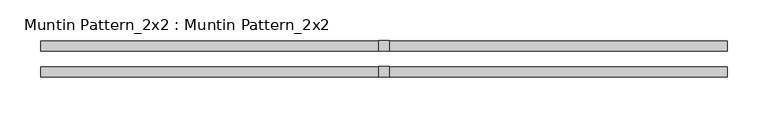
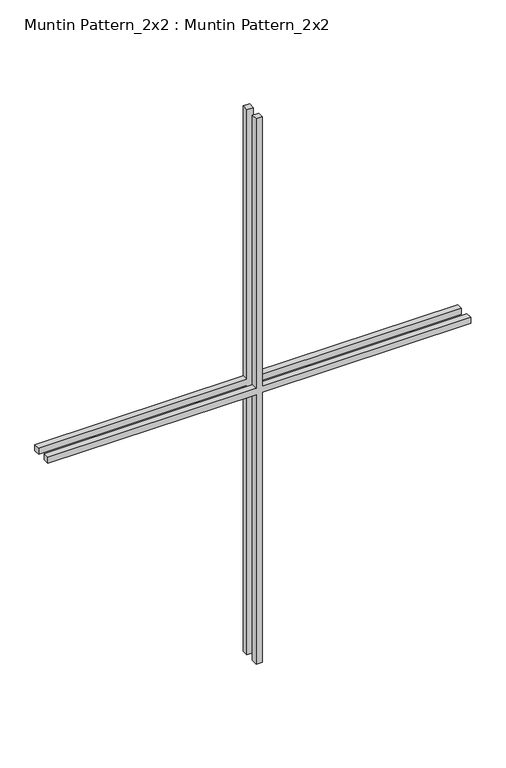
"""IFC4 building model written with IfcOpenShell, lengths in millimetres: proxy geometry, Muntin Pattern_2x2 : Muntin Pattern_2x2."""

import ifcopenshell
import ifcopenshell.guid

model = None  # the IFC model being written
_history = None  # IfcOwnerHistory: only IFC2X3 demands one
_inside = {}  # id of a spatial element -> (the spatial element, [elements in it])
_under = {}  # id of a project, library or spatial element -> (it, [spatial elements below it])
_declared = {}  # id of a project -> (the project, [libraries it declares])
_typed = {}  # id of a type object -> (the type object, [elements of that type])
_made_of = {}  # id of a material, layer set ... -> (it, [elements and type objects made of it])


def new_model(schema):
    """Start an empty IFC model of exactly this schema.

    Asked for "IFC4X3", IfcOpenShell would pick the latest addendum, in which some entities
    have other attributes; the version numbers below select the first issue.
    IFC2X3 requires an IfcOwnerHistory on every rooted entity: one is made here for all.
    """
    global model, _history
    if schema == "IFC4X3":
        model = ifcopenshell.file(schema_version=(4, 3, 0, 0))
    else:
        model = ifcopenshell.file(schema=schema)
    _inside.clear()
    _under.clear()
    _declared.clear()
    _typed.clear()
    _made_of.clear()
    _history = None
    if model.schema == "IFC2X3":
        org = make("IfcOrganization", Name="unknown")
        user = make(
            "IfcPersonAndOrganization",
            ThePerson=make("IfcPerson", FamilyName="unknown"),
            TheOrganization=org,
        )
        app = make(
            "IfcApplication",
            ApplicationDeveloper=org,
            Version="unknown",
            ApplicationFullName="unknown",
            ApplicationIdentifier="unknown",
        )
        _history = make(
            "IfcOwnerHistory",
            OwningUser=user,
            OwningApplication=app,
            ChangeAction="ADDED",
            CreationDate=0,
        )
    return model


def make(cls, **values):
    """One entity of the class cls with the attributes given. An attribute that is None is left unset."""
    return model.create_entity(
        cls, **{name: value for name, value in values.items() if value is not None}
    )


def rooted(cls, **values):
    """An entity with a GlobalId (a new one), such as an element, a storey or a relation."""
    return make(cls, GlobalId=ifcopenshell.guid.new(), OwnerHistory=_history, **values)


def si_unit(unit_type, name, prefix=None):
    """IfcSIUnit, for example si_unit("LENGTHUNIT", "METRE", prefix="MILLI")."""
    return make("IfcSIUnit", UnitType=unit_type, Prefix=prefix, Name=name)


def assignment(units):
    """IfcUnitAssignment: the units of a project."""
    return None if units is None else make("IfcUnitAssignment", Units=units)


def point(xyz):
    """IfcCartesianPoint."""
    return None if xyz is None else make("IfcCartesianPoint", Coordinates=xyz)


def direction(xyz):
    """IfcDirection."""
    return None if xyz is None else make("IfcDirection", DirectionRatios=xyz)


def frame(location, z_axis=None, x_axis=None):
    """IfcAxis2Placement3D, a coordinate frame: its origin and axes. An axis left out is left unset."""
    return make(
        "IfcAxis2Placement3D",
        Location=point(location),
        Axis=direction(z_axis),
        RefDirection=direction(x_axis),
    )


def origin():
    """The frame at (0, 0, 0) with its axes left unset."""
    return frame((0.0, 0.0, 0.0))


def place(relative_to, where):
    """IfcLocalPlacement: puts the frame where relative to a parent placement (None: the world)."""
    return make(
        "IfcLocalPlacement", PlacementRelTo=relative_to, RelativePlacement=where
    )


def context(
    kind, dimensions, precision=None, world=None, true_north=None, identifier=None
):
    """IfcGeometricRepresentationContext, for example the 3D "Model" context."""
    return make(
        "IfcGeometricRepresentationContext",
        ContextIdentifier=identifier,
        ContextType=kind,
        CoordinateSpaceDimension=dimensions,
        Precision=precision,
        WorldCoordinateSystem=world,
        TrueNorth=true_north,
    )


def project(units=None, contexts=None):
    """IfcProject with its units and contexts."""
    return rooted(
        "IfcProject",
        Name="project",
        RepresentationContexts=contexts,
        UnitsInContext=assignment(units),
    )


def spatial(cls, under=None, at=None, **own):
    """A site, building, storey or space (cls), placed at a placement, below another one or the project."""
    s = rooted(cls, ObjectPlacement=at, **own)
    if under is not None:
        _under.setdefault(under.id(), (under, []))[1].append(s)
    return s


def polyline(points):
    """IfcPolyline through the points."""
    return make("IfcPolyline", Points=[point(p) for p in points])


def outline(outer, holes=None, kind="AREA"):
    """IfcArbitraryClosedProfileDef: a profile drawn as a closed curve; with holes, ...WithVoids."""
    if holes is None:
        return make("IfcArbitraryClosedProfileDef", ProfileType=kind, OuterCurve=outer)
    return make(
        "IfcArbitraryProfileDefWithVoids",
        ProfileType=kind,
        OuterCurve=outer,
        InnerCurves=holes,
    )


def extrude(swept, where, along, depth):
    """IfcExtrudedAreaSolid: the profile swept, set in the frame where, extruded along a direction by depth."""
    return make(
        "IfcExtrudedAreaSolid",
        SweptArea=swept,
        Position=where,
        ExtrudedDirection=direction(along),
        Depth=depth,
    )


def shape(context_of_items, identifier, shape_type, items):
    """IfcShapeRepresentation: the items that make up one representation, for example the "Body"."""
    return make(
        "IfcShapeRepresentation",
        ContextOfItems=context_of_items,
        RepresentationIdentifier=identifier,
        RepresentationType=shape_type,
        Items=items,
    )


def source(mapping_origin, context_of_items, identifier, shape_type, items):
    """IfcRepresentationMap: a shape defined once, which mapped items show again and again."""
    return make(
        "IfcRepresentationMap",
        MappingOrigin=mapping_origin,
        MappedRepresentation=shape(context_of_items, identifier, shape_type, items),
    )


def transform(
    local_origin,
    x_axis=None,
    y_axis=None,
    z_axis=None,
    scale=None,
    scale2=None,
    scale3=None,
    uniform=True,
):
    """IfcCartesianTransformationOperator3D, or its non-uniform kind. x_axis, y_axis, z_axis: its Axis1, 2, 3."""
    if uniform:
        return make(
            "IfcCartesianTransformationOperator3D",
            Axis1=direction(x_axis),
            Axis2=direction(y_axis),
            LocalOrigin=point(local_origin),
            Scale=scale,
            Axis3=direction(z_axis),
        )
    return make(
        "IfcCartesianTransformationOperator3DnonUniform",
        Axis1=direction(x_axis),
        Axis2=direction(y_axis),
        LocalOrigin=point(local_origin),
        Scale=scale,
        Axis3=direction(z_axis),
        Scale2=scale2,
        Scale3=scale3,
    )


def mapped(mapping_source, mapping_target):
    """IfcMappedItem: shows the shape of a source again, moved by a transform."""
    return make(
        "IfcMappedItem", MappingSource=mapping_source, MappingTarget=mapping_target
    )


def made_of(thing, what):
    """Note that an element or type object is made of a material, layer set ...; save() writes the relation."""
    if what is not None:
        _made_of.setdefault(what.id(), (what, []))[1].append(thing)
    return thing


def element(
    cls,
    number,
    at=None,
    inside=None,
    cuts=None,
    type_object=None,
    material=None,
    context=None,
    identifier="Body",
    shape_type=None,
    held_by="IfcProductDefinitionShape",
    body=None,
    shapes=None,
    **own,
):
    """One element of the class cls, such as IfcWall. Its Tag is "e" and its number.

    at: its placement. inside: the storey or other place that contains it. cuts: it is an
    opening in that element (IfcRelVoidsElement). A single representation is given by context,
    identifier, shape_type and body (its items); several are given by shapes. held_by: the class
    of the entity that holds the representations. save() writes the other relations.
    """
    e = rooted(cls, Tag="e%d" % number, ObjectPlacement=at, **own)
    if body is not None:
        shapes = [shape(context, identifier, shape_type, body)]
    if shapes is not None:
        e.Representation = make(held_by, Representations=shapes)
    if inside is not None:
        _inside.setdefault(inside.id(), (inside, []))[1].append(e)
    if cuts is not None:
        rooted(
            "IfcRelVoidsElement", RelatingBuildingElement=cuts, RelatedOpeningElement=e
        )
    if type_object is not None:
        _typed.setdefault(type_object.id(), (type_object, []))[1].append(e)
    return made_of(e, material)


def aggregate(whole, parts):
    """IfcRelAggregates: a whole, such as a stair, and the parts it consists of."""
    return rooted("IfcRelAggregates", RelatingObject=whole, RelatedObjects=parts)


def save(model, path):
    """Write the relations noted so far, then the file.

    IfcRelAggregates (storeys below a building ...), IfcRelContainedInSpatialStructure (elements
    in a storey), IfcRelDefinesByType, IfcRelAssociatesMaterial and IfcRelDeclares: one each for
    every whole, place, type object, material and project.
    """
    for whole, parts in _under.values():
        aggregate(whole, parts)
    for where, things in _inside.values():
        rooted(
            "IfcRelContainedInSpatialStructure",
            RelatedElements=things,
            RelatingStructure=where,
        )
    for kind, things in _typed.values():
        rooted("IfcRelDefinesByType", RelatedObjects=things, RelatingType=kind)
    for what, things in _made_of.values():
        rooted("IfcRelAssociatesMaterial", RelatedObjects=things, RelatingMaterial=what)
    for by, libraries in _declared.values():
        rooted("IfcRelDeclares", RelatingContext=by, RelatedDefinitions=libraries)
    model.write(path)


def muntin_pattern_2x2_muntin_pattern_2x2_0b2f62cf(model_context):
    return source(origin(), model_context, "Body", "SweptSolid", [
        extrude(outline(polyline([(577.85, -6.35), (577.85, -419.1), (565.15, -419.1), (565.15, -6.35), (0.0, -6.35), (0.0, 6.35), (565.15, 6.35), (565.15, 419.1), (577.85, 419.1), (577.85, 6.35), (1143.0, 6.35), (1143.0, -6.35), (577.85, -6.35)])), frame((0.0, -22.225, 0.0), z_axis=(0.0, 1.0, 0.0), x_axis=(0.0, 0.0, 1.0)), (0.0, 0.0, 1.0), 12.7),
        extrude(outline(polyline([(577.85, -6.35), (577.85, -419.1), (565.15, -419.1), (565.15, -6.35), (0.0, -6.35), (0.0, 6.35), (565.15, 6.35), (565.15, 419.1), (577.85, 419.1), (577.85, 6.35), (1143.0, 6.35), (1143.0, -6.35), (577.85, -6.35)])), frame((0.0, 9.525, 0.0), z_axis=(0.0, 1.0, 0.0), x_axis=(0.0, 0.0, 1.0)), (0.0, 0.0, 1.0), 12.7),
    ])


if __name__ == "__main__":
    model = new_model("IFC4")
    model_context = context("Model", 3, world=origin())
    ifc_project = project(units=[si_unit("LENGTHUNIT", "METRE", prefix="MILLI")], contexts=[model_context])
    site = spatial("IfcSite", under=ifc_project)
    building = spatial("IfcBuilding", under=site)
    placement = place(None, origin())
    muntin_pattern_2x2_muntin_pattern_2x2_shape = muntin_pattern_2x2_muntin_pattern_2x2_0b2f62cf(model_context)
    element("IfcBuildingElementProxy", 1, Name="Muntin Pattern_2x2 : Muntin Pattern_2x2", ObjectType="Muntin Pattern_2x2 : Muntin Pattern_2x2", at=placement, inside=building, context=model_context, shape_type="MappedRepresentation", body=[
        mapped(muntin_pattern_2x2_muntin_pattern_2x2_shape, transform((0.0, 0.0, 0.0), x_axis=(1.0, 0.0, 0.0), y_axis=(0.0, 1.0, 0.0), z_axis=(0.0, 0.0, 1.0))),
    ])
    save(model, "model.ifc")

# Revit data of these elements
# Type "Muntin Pattern_2x2 : Muntin Pattern_2x2"
#   Width [instance default] = 4.00 ft
#   Thickness = 0.041667 ft
#   Height [instance default] = 4.00 ft
#   Distance = 0.0625 ft
#   Interior Material [instance default] = none
#   Exterior Material [instance default] = none
#   Default Elevation = 0
# Element 1 (IfcBuildingElementProxy, "Muntin Pattern_2x2 : Muntin Pattern_2x2")
#   Width = 2.75 ft
#   Height = 3.75 ft
#   Interior Material = Maple - Semigloss
#   Exterior Material = Clad - White
#   Materials on its faces: "Clad - White", "Maple - Semigloss"
# Materials
#   "Clad - White": class "Wood", colour RGB 245 245 243, transparency 0, Cost = 0
#   "Maple - Semigloss": class "Wood", colour RGB 196 161 118, transparency 0, Description = "Acer Saccharum", Cost = 0
